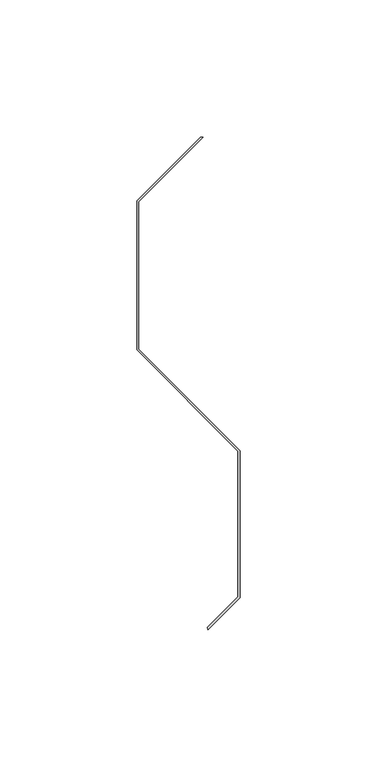
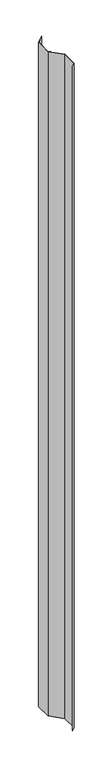
"""IFC4 building model written with IfcOpenShell, lengths in millimetres: proxy geometry, MBCI 7.2-V Panel40 : MBCI 7.2-V Panel-1."""

import ifcopenshell
import ifcopenshell.guid

model = None  # the IFC model being written
_history = None  # IfcOwnerHistory: only IFC2X3 demands one
_inside = {}  # id of a spatial element -> (the spatial element, [elements in it])
_under = {}  # id of a project, library or spatial element -> (it, [spatial elements below it])
_declared = {}  # id of a project -> (the project, [libraries it declares])
_typed = {}  # id of a type object -> (the type object, [elements of that type])
_made_of = {}  # id of a material, layer set ... -> (it, [elements and type objects made of it])


def new_model(schema):
    """Start an empty IFC model of exactly this schema.

    Asked for "IFC4X3", IfcOpenShell would pick the latest addendum, in which some entities
    have other attributes; the version numbers below select the first issue.
    IFC2X3 requires an IfcOwnerHistory on every rooted entity: one is made here for all.
    """
    global model, _history
    if schema == "IFC4X3":
        model = ifcopenshell.file(schema_version=(4, 3, 0, 0))
    else:
        model = ifcopenshell.file(schema=schema)
    _inside.clear()
    _under.clear()
    _declared.clear()
    _typed.clear()
    _made_of.clear()
    _history = None
    if model.schema == "IFC2X3":
        org = make("IfcOrganization", Name="unknown")
        user = make(
            "IfcPersonAndOrganization",
            ThePerson=make("IfcPerson", FamilyName="unknown"),
            TheOrganization=org,
        )
        app = make(
            "IfcApplication",
            ApplicationDeveloper=org,
            Version="unknown",
            ApplicationFullName="unknown",
            ApplicationIdentifier="unknown",
        )
        _history = make(
            "IfcOwnerHistory",
            OwningUser=user,
            OwningApplication=app,
            ChangeAction="ADDED",
            CreationDate=0,
        )
    return model


def make(cls, **values):
    """One entity of the class cls with the attributes given. An attribute that is None is left unset."""
    return model.create_entity(
        cls, **{name: value for name, value in values.items() if value is not None}
    )


def rooted(cls, **values):
    """An entity with a GlobalId (a new one), such as an element, a storey or a relation."""
    return make(cls, GlobalId=ifcopenshell.guid.new(), OwnerHistory=_history, **values)


def si_unit(unit_type, name, prefix=None):
    """IfcSIUnit, for example si_unit("LENGTHUNIT", "METRE", prefix="MILLI")."""
    return make("IfcSIUnit", UnitType=unit_type, Prefix=prefix, Name=name)


def assignment(units):
    """IfcUnitAssignment: the units of a project."""
    return None if units is None else make("IfcUnitAssignment", Units=units)


def point(xyz):
    """IfcCartesianPoint."""
    return None if xyz is None else make("IfcCartesianPoint", Coordinates=xyz)


def direction(xyz):
    """IfcDirection."""
    return None if xyz is None else make("IfcDirection", DirectionRatios=xyz)


def frame(location, z_axis=None, x_axis=None):
    """IfcAxis2Placement3D, a coordinate frame: its origin and axes. An axis left out is left unset."""
    return make(
        "IfcAxis2Placement3D",
        Location=point(location),
        Axis=direction(z_axis),
        RefDirection=direction(x_axis),
    )


def origin():
    """The frame at (0, 0, 0) with its axes left unset."""
    return frame((0.0, 0.0, 0.0))


def place(relative_to, where):
    """IfcLocalPlacement: puts the frame where relative to a parent placement (None: the world)."""
    return make(
        "IfcLocalPlacement", PlacementRelTo=relative_to, RelativePlacement=where
    )


def context(
    kind, dimensions, precision=None, world=None, true_north=None, identifier=None
):
    """IfcGeometricRepresentationContext, for example the 3D "Model" context."""
    return make(
        "IfcGeometricRepresentationContext",
        ContextIdentifier=identifier,
        ContextType=kind,
        CoordinateSpaceDimension=dimensions,
        Precision=precision,
        WorldCoordinateSystem=world,
        TrueNorth=true_north,
    )


def project(units=None, contexts=None):
    """IfcProject with its units and contexts."""
    return rooted(
        "IfcProject",
        Name="project",
        RepresentationContexts=contexts,
        UnitsInContext=assignment(units),
    )


def spatial(cls, under=None, at=None, **own):
    """A site, building, storey or space (cls), placed at a placement, below another one or the project."""
    s = rooted(cls, ObjectPlacement=at, **own)
    if under is not None:
        _under.setdefault(under.id(), (under, []))[1].append(s)
    return s


def polyline(points):
    """IfcPolyline through the points."""
    return make("IfcPolyline", Points=[point(p) for p in points])


def outline(outer, holes=None, kind="AREA"):
    """IfcArbitraryClosedProfileDef: a profile drawn as a closed curve; with holes, ...WithVoids."""
    if holes is None:
        return make("IfcArbitraryClosedProfileDef", ProfileType=kind, OuterCurve=outer)
    return make(
        "IfcArbitraryProfileDefWithVoids",
        ProfileType=kind,
        OuterCurve=outer,
        InnerCurves=holes,
    )


def extrude(swept, where, along, depth):
    """IfcExtrudedAreaSolid: the profile swept, set in the frame where, extruded along a direction by depth."""
    return make(
        "IfcExtrudedAreaSolid",
        SweptArea=swept,
        Position=where,
        ExtrudedDirection=direction(along),
        Depth=depth,
    )


def shape(context_of_items, identifier, shape_type, items):
    """IfcShapeRepresentation: the items that make up one representation, for example the "Body"."""
    return make(
        "IfcShapeRepresentation",
        ContextOfItems=context_of_items,
        RepresentationIdentifier=identifier,
        RepresentationType=shape_type,
        Items=items,
    )


def source(mapping_origin, context_of_items, identifier, shape_type, items):
    """IfcRepresentationMap: a shape defined once, which mapped items show again and again."""
    return make(
        "IfcRepresentationMap",
        MappingOrigin=mapping_origin,
        MappedRepresentation=shape(context_of_items, identifier, shape_type, items),
    )


def transform(
    local_origin,
    x_axis=None,
    y_axis=None,
    z_axis=None,
    scale=None,
    scale2=None,
    scale3=None,
    uniform=True,
):
    """IfcCartesianTransformationOperator3D, or its non-uniform kind. x_axis, y_axis, z_axis: its Axis1, 2, 3."""
    if uniform:
        return make(
            "IfcCartesianTransformationOperator3D",
            Axis1=direction(x_axis),
            Axis2=direction(y_axis),
            LocalOrigin=point(local_origin),
            Scale=scale,
            Axis3=direction(z_axis),
        )
    return make(
        "IfcCartesianTransformationOperator3DnonUniform",
        Axis1=direction(x_axis),
        Axis2=direction(y_axis),
        LocalOrigin=point(local_origin),
        Scale=scale,
        Axis3=direction(z_axis),
        Scale2=scale2,
        Scale3=scale3,
    )


def mapped(mapping_source, mapping_target):
    """IfcMappedItem: shows the shape of a source again, moved by a transform."""
    return make(
        "IfcMappedItem", MappingSource=mapping_source, MappingTarget=mapping_target
    )


def made_of(thing, what):
    """Note that an element or type object is made of a material, layer set ...; save() writes the relation."""
    if what is not None:
        _made_of.setdefault(what.id(), (what, []))[1].append(thing)
    return thing


def element(
    cls,
    number,
    at=None,
    inside=None,
    cuts=None,
    type_object=None,
    material=None,
    context=None,
    identifier="Body",
    shape_type=None,
    held_by="IfcProductDefinitionShape",
    body=None,
    shapes=None,
    **own,
):
    """One element of the class cls, such as IfcWall. Its Tag is "e" and its number.

    at: its placement. inside: the storey or other place that contains it. cuts: it is an
    opening in that element (IfcRelVoidsElement). A single representation is given by context,
    identifier, shape_type and body (its items); several are given by shapes. held_by: the class
    of the entity that holds the representations. save() writes the other relations.
    """
    e = rooted(cls, Tag="e%d" % number, ObjectPlacement=at, **own)
    if body is not None:
        shapes = [shape(context, identifier, shape_type, body)]
    if shapes is not None:
        e.Representation = make(held_by, Representations=shapes)
    if inside is not None:
        _inside.setdefault(inside.id(), (inside, []))[1].append(e)
    if cuts is not None:
        rooted(
            "IfcRelVoidsElement", RelatingBuildingElement=cuts, RelatedOpeningElement=e
        )
    if type_object is not None:
        _typed.setdefault(type_object.id(), (type_object, []))[1].append(e)
    return made_of(e, material)


def aggregate(whole, parts):
    """IfcRelAggregates: a whole, such as a stair, and the parts it consists of."""
    return rooted("IfcRelAggregates", RelatingObject=whole, RelatedObjects=parts)


def save(model, path):
    """Write the relations noted so far, then the file.

    IfcRelAggregates (storeys below a building ...), IfcRelContainedInSpatialStructure (elements
    in a storey), IfcRelDefinesByType, IfcRelAssociatesMaterial and IfcRelDeclares: one each for
    every whole, place, type object, material and project.
    """
    for whole, parts in _under.values():
        aggregate(whole, parts)
    for where, things in _inside.values():
        rooted(
            "IfcRelContainedInSpatialStructure",
            RelatedElements=things,
            RelatingStructure=where,
        )
    for kind, things in _typed.values():
        rooted("IfcRelDefinesByType", RelatedObjects=things, RelatingType=kind)
    for what, things in _made_of.values():
        rooted("IfcRelAssociatesMaterial", RelatedObjects=things, RelatingMaterial=what)
    for by, libraries in _declared.values():
        rooted("IfcRelDeclares", RelatingContext=by, RelatedDefinitions=libraries)
    model.write(path)


def generic_models_065db151(model_context):
    return source(origin(), model_context, "Body", "SweptSolid", [
        extrude(outline(polyline([(587365.2695864, -535322.081684), (587365.2695864, -535375.662984), (587353.5988637, -535387.3337068), (587353.54384, -535386.5468314), (587364.6742739, -535375.4163975), (587364.6742739, -535322.3282706), (587327.7791864, -535285.4331831), (587327.7791864, -535231.1525192), (587351.0153216, -535207.9163841), (587351.8572206, -535207.9163841), (587328.3744989, -535231.3991057), (587328.3744989, -535285.1865965), (587365.2695864, -535322.081684)])), frame((0.0, 0.0, 51.59375), z_axis=(0.0, 0.0, 1.0), x_axis=(1.0, 0.0, 0.0)), (0.0, 0.0, 1.0), 2386.80625),
    ])


if __name__ == "__main__":
    model = new_model("IFC4")
    model_context = context("Model", 3, world=origin())
    ifc_project = project(units=[si_unit("LENGTHUNIT", "METRE", prefix="MILLI")], contexts=[model_context])
    site = spatial("IfcSite", under=ifc_project)
    building = spatial("IfcBuilding", under=site)
    placement = place(None, origin())
    generic_models_shape = generic_models_065db151(model_context)
    element("IfcBuildingElementProxy", 1, Name="MBCI 7.2-V Panel40 : MBCI 7.2-V Panel-1", ObjectType="MBCI 7.2-V Panel40 : MBCI 7.2-V Panel-1", at=placement, inside=building, context=model_context, shape_type="MappedRepresentation", body=[
        mapped(generic_models_shape, transform((0.0, 0.0, 0.0), x_axis=(1.0, 0.0, 0.0), y_axis=(0.0, 1.0, 0.0), z_axis=(0.0, 0.0, 1.0))),
    ])
    save(model, "model.ifc")

# Revit data of these elements
# Element 1 (IfcBuildingElementProxy, "MBCI 7.2-V Panel40 : MBCI 7.2-V Panel-1")
#   Materials on its faces: "MTL PANEL"
# Materials
#   "MTL PANEL": class "Generic", colour RGB 239 242 240, transparency 0, Cost = 0
